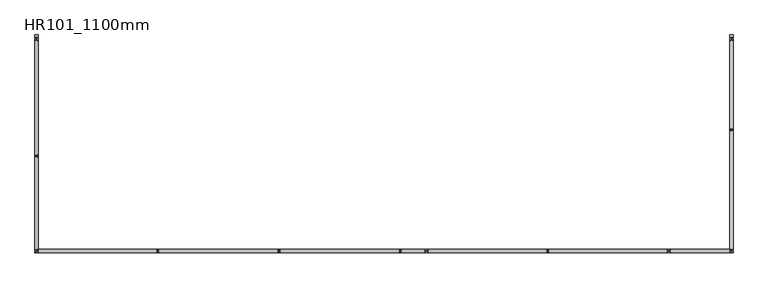
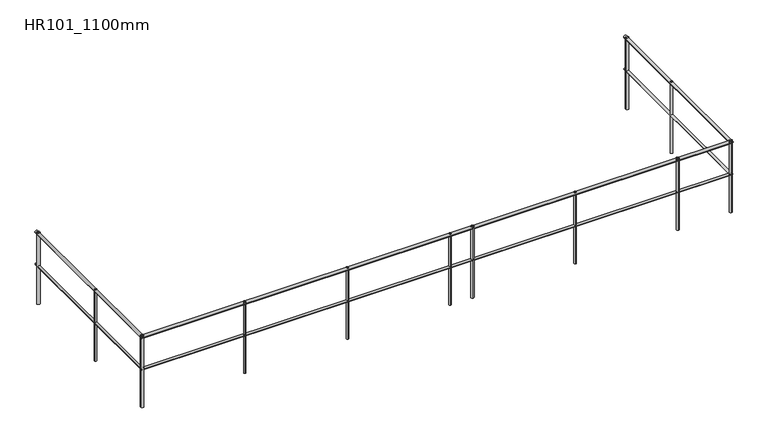
"""IFC4 building model written with IfcOpenShell, lengths in millimetres: railing geometry, HR101_1100mm."""

from ifc_helpers import new_model, si_unit, point, frame, frame_2d, origin, place, context, project, spatial, circle_curve, ellipse_curve, trimmed, segment, composite_curve, outline, extrude, source, transform, mapped, element, save
from ifc_brep_helpers import plane_surface, cylinder_surface, advanced_brep


def hr101_1100mm_0ef6d300(model_context):
    return source(origin(), model_context, "Body", "SolidModel", [
        advanced_brep(
        [(-308.0, 20699.5208589, 5133.005241), (-342.0, 20699.5208589, 5133.005241), (-308.0, 18041.5208589, 5133.005241), (-342.0, 18007.5208589, 5133.005241), (8258.0, 18041.5208589, 5133.005241), (8292.0, 18007.5208589, 5133.005241), (8258.0, 20699.5208589, 5133.005241), (8292.0, 20699.5208589, 5133.005241)],
        [
            (0, 1, circle_curve(frame((-325.0, 20699.5208589, 5133.005241), z_axis=(0.0, 1.0, 0.0), x_axis=(-1.0, 0.0, 0.0)), 17.0)),
            (1, 0, circle_curve(frame((-325.0, 20699.5208589, 5133.005241), z_axis=(0.0, 1.0, 0.0), x_axis=(-1.0, 0.0, 0.0)), 17.0)),
            (0, 2),
            (2, 3, ellipse_curve(frame((-325.0, 18024.5208589, 5133.005241), z_axis=(-0.7071067811865475, 0.7071067811865475, 0.0), x_axis=(0.7071067811865474, 0.7071067811865476, 0.0)), 24.0416306, 17.0)),
            (3, 1),
            (3, 2, ellipse_curve(frame((-325.0, 18024.5208589, 5133.005241), z_axis=(-0.7071067811865475, 0.7071067811865475, 0.0), x_axis=(0.7071067811865474, 0.7071067811865476, 0.0)), 24.0416306, 17.0)),
            (2, 4),
            (4, 5, ellipse_curve(frame((8275.0, 18024.5208589, 5133.005241), z_axis=(-0.7071067811865475, -0.7071067811865475, 0.0), x_axis=(-0.7071067811865476, 0.7071067811865474, 0.0)), 24.0416306, 17.0)),
            (5, 3),
            (5, 4, ellipse_curve(frame((8275.0, 18024.5208589, 5133.005241), z_axis=(-0.7071067811865475, -0.7071067811865475, 0.0), x_axis=(-0.7071067811865476, 0.7071067811865474, 0.0)), 24.0416306, 17.0)),
            (6, 7, circle_curve(frame((8275.0, 20699.5208589, 5133.005241), z_axis=(0.0, 1.0, 0.0), x_axis=(1.0, 0.0, 0.0)), 17.0)),
            (7, 6, circle_curve(frame((8275.0, 20699.5208589, 5133.005241), z_axis=(0.0, 1.0, 0.0), x_axis=(1.0, 0.0, 0.0)), 17.0)),
            (4, 6),
            (7, 5),
        ],
        [
            plane_surface(frame((-325.0, 20699.5208589, 5150.005241), z_axis=(0.0, 1.0, 0.0), x_axis=(0.0, 0.0, -1.0))),
            cylinder_surface(frame((-325.0, 20699.5208589, 5133.005241), z_axis=(0.0, 1.0, 0.0), x_axis=(-1.0, 0.0, 0.0)), 17.0),
            cylinder_surface(frame((-325.0, 18024.5208589, 5133.005241), z_axis=(-1.0, 0.0, 0.0), x_axis=(0.0, -1.0, 0.0)), 17.0),
            plane_surface(frame((8275.0, 20699.5208589, 5150.005241), z_axis=(0.0, 1.0, 0.0), x_axis=(0.0, 0.0, 1.0))),
            cylinder_surface(frame((8275.0, 18024.5208589, 5133.005241), z_axis=(0.0, -1.0, 0.0), x_axis=(1.0, 0.0, 0.0)), 17.0),
        ],
        [
            (0, [[1, 2]]),
            (1, [[-1, 3, 4, 5]]),
            (1, [[-2, -5, 6, -3]]),
            (2, [[-4, 7, 8, 9]]),
            (2, [[-6, -9, 10, -7]]),
            (3, [[11, 12]]),
            (4, [[-8, 13, -12, 14]]),
            (4, [[-10, -14, -11, -13]]),
        ],
    ),
        advanced_brep(
        [(-303.65, 20699.5208589, 5628.655241), (-346.35, 20699.5208589, 5628.655241), (-303.65, 18045.8708589, 5628.655241), (-346.35, 18003.1708589, 5628.655241), (8253.65, 18045.8708589, 5628.655241), (8296.35, 18003.1708589, 5628.655241), (8253.65, 20699.5208589, 5628.655241), (8296.35, 20699.5208589, 5628.655241)],
        [
            (0, 1, circle_curve(frame((-325.0, 20699.5208589, 5628.655241), z_axis=(0.0, 1.0, 0.0), x_axis=(-1.0, 0.0, 0.0)), 21.35)),
            (1, 0, circle_curve(frame((-325.0, 20699.5208589, 5628.655241), z_axis=(0.0, 1.0, 0.0), x_axis=(-1.0, 0.0, 0.0)), 21.35)),
            (0, 2),
            (2, 3, ellipse_curve(frame((-325.0, 18024.5208589, 5628.655241), z_axis=(-0.7071067811865475, 0.7071067811865475, 0.0), x_axis=(0.7071067811865474, 0.7071067811865476, 0.0)), 30.1934596, 21.35)),
            (3, 1),
            (3, 2, ellipse_curve(frame((-325.0, 18024.5208589, 5628.655241), z_axis=(-0.7071067811865475, 0.7071067811865475, 0.0), x_axis=(0.7071067811865474, 0.7071067811865476, 0.0)), 30.1934596, 21.35)),
            (2, 4),
            (4, 5, ellipse_curve(frame((8275.0, 18024.5208589, 5628.655241), z_axis=(-0.7071067811865475, -0.7071067811865475, 0.0), x_axis=(-0.7071067811865476, 0.7071067811865474, 0.0)), 30.1934596, 21.35)),
            (5, 3),
            (5, 4, ellipse_curve(frame((8275.0, 18024.5208589, 5628.655241), z_axis=(-0.7071067811865475, -0.7071067811865475, 0.0), x_axis=(-0.7071067811865476, 0.7071067811865474, 0.0)), 30.1934596, 21.35)),
            (6, 7, circle_curve(frame((8275.0, 20699.5208589, 5628.655241), z_axis=(0.0, 1.0, 0.0), x_axis=(1.0, 0.0, 0.0)), 21.35)),
            (7, 6, circle_curve(frame((8275.0, 20699.5208589, 5628.655241), z_axis=(0.0, 1.0, 0.0), x_axis=(1.0, 0.0, 0.0)), 21.35)),
            (4, 6),
            (7, 5),
        ],
        [
            plane_surface(frame((-325.0, 20699.5208589, 5650.005241), z_axis=(0.0, 1.0, 0.0), x_axis=(0.0, 0.0, -1.0))),
            cylinder_surface(frame((-325.0, 20699.5208589, 5628.655241), z_axis=(0.0, 1.0, 0.0), x_axis=(-1.0, 0.0, 0.0)), 21.35),
            cylinder_surface(frame((-325.0, 18024.5208589, 5628.655241), z_axis=(-1.0, 0.0, 0.0), x_axis=(0.0, -1.0, 0.0)), 21.35),
            plane_surface(frame((8275.0, 20699.5208589, 5650.005241), z_axis=(0.0, 1.0, 0.0), x_axis=(0.0, 0.0, 1.0))),
            cylinder_surface(frame((8275.0, 18024.5208589, 5628.655241), z_axis=(0.0, -1.0, 0.0), x_axis=(1.0, 0.0, 0.0)), 21.35),
        ],
        [
            (0, [[1, 2]]),
            (1, [[-1, 3, 4, 5]]),
            (1, [[-2, -5, 6, -3]]),
            (2, [[-4, 7, 8, 9]]),
            (2, [[-6, -9, 10, -7]]),
            (3, [[11, 12]]),
            (4, [[-8, 13, -12, 14]]),
            (4, [[-10, -14, -11, -13]]),
        ],
    ),
        extrude(outline(composite_curve([segment(trimmed(circle_curve(frame_2d((8275.0, 19524.5208589)), 15.0), [point((8290.0, 19524.5208589))], [point((8260.0, 19524.5208589))], False, "CARTESIAN"), True, "CONTINUOUS"), segment(trimmed(circle_curve(frame_2d((8275.0, 19524.5208589)), 15.0), [point((8260.0, 19524.5208589))], [point((8290.0, 19524.5208589))], False, "CARTESIAN"), True, "CONTINUOUS")], self_intersect=False)), frame((0.0, 0.0, 4550.005241), z_axis=(0.0, 0.0, 1.0), x_axis=(1.0, 0.0, 0.0)), (0.0, 0.0, 1.0), 1100.0),
        extrude(outline(composite_curve([segment(trimmed(circle_curve(frame_2d((6000.0, 18024.5208589)), 15.0), [point((6000.0, 18009.5208589))], [point((6000.0, 18039.5208589))], False, "CARTESIAN"), True, "CONTINUOUS"), segment(trimmed(circle_curve(frame_2d((6000.0, 18024.5208589)), 15.0), [point((6000.0, 18039.5208589))], [point((6000.0, 18009.5208589))], False, "CARTESIAN"), True, "CONTINUOUS")], self_intersect=False)), frame((0.0, 0.0, 4550.005241), z_axis=(0.0, 0.0, 1.0), x_axis=(1.0, 0.0, 0.0)), (0.0, 0.0, 1.0), 1100.0),
        extrude(outline(composite_curve([segment(trimmed(circle_curve(frame_2d((4175.0, 18024.5208589)), 15.0), [point((4175.0, 18009.5208589))], [point((4175.0, 18039.5208589))], False, "CARTESIAN"), True, "CONTINUOUS"), segment(trimmed(circle_curve(frame_2d((4175.0, 18024.5208589)), 15.0), [point((4175.0, 18039.5208589))], [point((4175.0, 18009.5208589))], False, "CARTESIAN"), True, "CONTINUOUS")], self_intersect=False)), frame((0.0, 0.0, 4550.005241), z_axis=(0.0, 0.0, 1.0), x_axis=(1.0, 0.0, 0.0)), (0.0, 0.0, 1.0), 1100.0),
        extrude(outline(composite_curve([segment(trimmed(circle_curve(frame_2d((2675.0, 18024.5208589)), 15.0), [point((2675.0, 18009.5208589))], [point((2675.0, 18039.5208589))], False, "CARTESIAN"), True, "CONTINUOUS"), segment(trimmed(circle_curve(frame_2d((2675.0, 18024.5208589)), 15.0), [point((2675.0, 18039.5208589))], [point((2675.0, 18009.5208589))], False, "CARTESIAN"), True, "CONTINUOUS")], self_intersect=False)), frame((0.0, 0.0, 4550.005241), z_axis=(0.0, 0.0, 1.0), x_axis=(1.0, 0.0, 0.0)), (0.0, 0.0, 1.0), 1100.0),
        extrude(outline(composite_curve([segment(trimmed(circle_curve(frame_2d((1175.0, 18024.5208589)), 15.0), [point((1175.0, 18009.5208589))], [point((1175.0, 18039.5208589))], False, "CARTESIAN"), True, "CONTINUOUS"), segment(trimmed(circle_curve(frame_2d((1175.0, 18024.5208589)), 15.0), [point((1175.0, 18039.5208589))], [point((1175.0, 18009.5208589))], False, "CARTESIAN"), True, "CONTINUOUS")], self_intersect=False)), frame((0.0, 0.0, 4550.005241), z_axis=(0.0, 0.0, 1.0), x_axis=(1.0, 0.0, 0.0)), (0.0, 0.0, 1.0), 1100.0),
        extrude(outline(composite_curve([segment(trimmed(circle_curve(frame_2d((-325.0, 19199.5208589)), 15.0), [point((-340.0, 19199.5208589))], [point((-310.0, 19199.5208589))], False, "CARTESIAN"), True, "CONTINUOUS"), segment(trimmed(circle_curve(frame_2d((-325.0, 19199.5208589)), 15.0), [point((-310.0, 19199.5208589))], [point((-340.0, 19199.5208589))], False, "CARTESIAN"), True, "CONTINUOUS")], self_intersect=False)), frame((0.0, 0.0, 4550.005241), z_axis=(0.0, 0.0, 1.0), x_axis=(1.0, 0.0, 0.0)), (0.0, 0.0, 1.0), 1100.0),
        extrude(outline(composite_curve([segment(trimmed(circle_curve(frame_2d((8275.0, 18024.5208589)), 21.35), [point((8275.0, 18003.1708589))], [point((8275.0, 18045.8708589))], False, "CARTESIAN"), True, "CONTINUOUS"), segment(trimmed(circle_curve(frame_2d((8275.0, 18024.5208589)), 21.35), [point((8275.0, 18045.8708589))], [point((8275.0, 18003.1708589))], False, "CARTESIAN"), True, "CONTINUOUS")], self_intersect=False)), frame((0.0, 0.0, 4550.005241), z_axis=(0.0, 0.0, 1.0), x_axis=(1.0, 0.0, 0.0)), (0.0, 0.0, 1.0), 1100.0),
        extrude(outline(composite_curve([segment(trimmed(circle_curve(frame_2d((7500.0, 18024.5208589)), 21.35), [point((7500.0, 18003.1708589))], [point((7500.0, 18045.8708589))], False, "CARTESIAN"), True, "CONTINUOUS"), segment(trimmed(circle_curve(frame_2d((7500.0, 18024.5208589)), 21.35), [point((7500.0, 18045.8708589))], [point((7500.0, 18003.1708589))], False, "CARTESIAN"), True, "CONTINUOUS")], self_intersect=False)), frame((0.0, 0.0, 4550.005241), z_axis=(0.0, 0.0, 1.0), x_axis=(1.0, 0.0, 0.0)), (0.0, 0.0, 1.0), 1100.0),
        extrude(outline(composite_curve([segment(trimmed(circle_curve(frame_2d((4500.0, 18024.5208589)), 21.35), [point((4500.0, 18003.1708589))], [point((4500.0, 18045.8708589))], False, "CARTESIAN"), True, "CONTINUOUS"), segment(trimmed(circle_curve(frame_2d((4500.0, 18024.5208589)), 21.35), [point((4500.0, 18045.8708589))], [point((4500.0, 18003.1708589))], False, "CARTESIAN"), True, "CONTINUOUS")], self_intersect=False)), frame((0.0, 0.0, 4550.005241), z_axis=(0.0, 0.0, 1.0), x_axis=(1.0, 0.0, 0.0)), (0.0, 0.0, 1.0), 1100.0),
        extrude(outline(composite_curve([segment(trimmed(circle_curve(frame_2d((-325.0, 18024.5208589)), 21.35), [point((-346.35, 18024.5208589))], [point((-303.65, 18024.5208589))], False, "CARTESIAN"), True, "CONTINUOUS"), segment(trimmed(circle_curve(frame_2d((-325.0, 18024.5208589)), 21.35), [point((-303.65, 18024.5208589))], [point((-346.35, 18024.5208589))], False, "CARTESIAN"), True, "CONTINUOUS")], self_intersect=False)), frame((0.0, 0.0, 4550.005241), z_axis=(0.0, 0.0, 1.0), x_axis=(1.0, 0.0, 0.0)), (0.0, 0.0, 1.0), 1100.0),
        extrude(outline(composite_curve([segment(trimmed(circle_curve(frame_2d((8275.0, 20649.5208589)), 21.35), [point((8296.35, 20649.5208589))], [point((8253.65, 20649.5208589))], False, "CARTESIAN"), True, "CONTINUOUS"), segment(trimmed(circle_curve(frame_2d((8275.0, 20649.5208589)), 21.35), [point((8253.65, 20649.5208589))], [point((8296.35, 20649.5208589))], False, "CARTESIAN"), True, "CONTINUOUS")], self_intersect=False)), frame((0.0, 0.0, 4550.005241), z_axis=(0.0, 0.0, 1.0), x_axis=(1.0, 0.0, 0.0)), (0.0, 0.0, 1.0), 1100.0),
        extrude(outline(composite_curve([segment(trimmed(circle_curve(frame_2d((-325.0, 20649.5208589)), 21.35), [point((-346.35, 20649.5208589))], [point((-303.65, 20649.5208589))], False, "CARTESIAN"), True, "CONTINUOUS"), segment(trimmed(circle_curve(frame_2d((-325.0, 20649.5208589)), 21.35), [point((-303.65, 20649.5208589))], [point((-346.35, 20649.5208589))], False, "CARTESIAN"), True, "CONTINUOUS")], self_intersect=False)), frame((0.0, 0.0, 4550.005241), z_axis=(0.0, 0.0, 1.0), x_axis=(1.0, 0.0, 0.0)), (0.0, 0.0, 1.0), 1100.0),
    ])


if __name__ == "__main__":
    model = new_model("IFC4")
    model_context = context("Model", 3, world=origin())
    ifc_project = project(units=[si_unit("LENGTHUNIT", "METRE", prefix="MILLI")], contexts=[model_context])
    site = spatial("IfcSite", under=ifc_project)
    building = spatial("IfcBuilding", under=site)
    placement = place(None, origin())
    hr101_1100mm_shape = hr101_1100mm_0ef6d300(model_context)
    element("IfcRailing", 1, ObjectType="HR101_1100mm", at=placement, inside=building, context=model_context, shape_type="MappedRepresentation", body=[
        mapped(hr101_1100mm_shape, transform((0.0, 0.0, 0.0), x_axis=(1.0, 0.0, 0.0), y_axis=(0.0, 1.0, 0.0), z_axis=(0.0, 0.0, 1.0))),
    ])
    save(model, "model.ifc")

# Revit data of these elements
# Element 1 (IfcRailing, "HR101_1100mm")
#   Materials on its faces: "S02AA020-00001_Steel Handrails"
# Materials
#   "S02AA020-00001_Steel Handrails": class "Metal", colour RGB 148 148 148, transparency 0, Description = "STEEL HANDRAIL(TYP.)", Cost = 0
